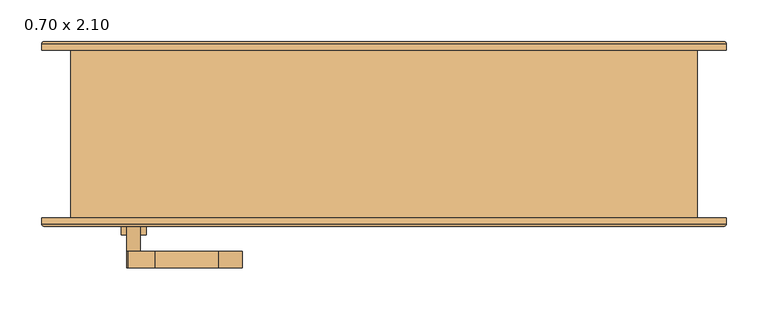
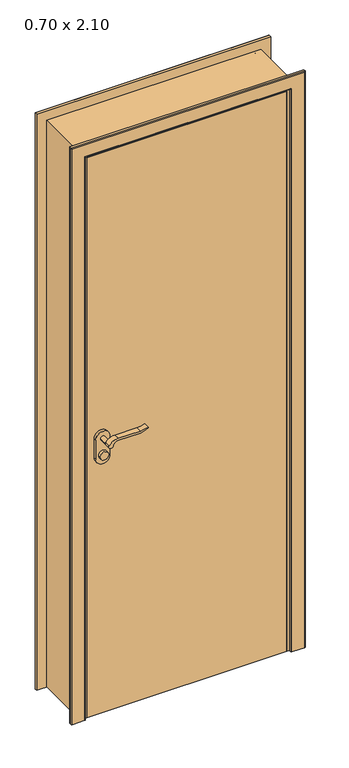
"""IFC4 building model written with IfcOpenShell, lengths in millimetres: door geometry, .CC_ND 300_PORTA SIMPLES DE ABRIR_COM EXTENSÃO : 0.70 x 2.10."""

from ifc_helpers import new_model, si_unit, point, frame, frame_2d, origin, origin_with_axes, place, context, project, spatial, polyline, circle_curve, ellipse_curve, trimmed, segment, composite_curve, outline, extrude, faceted_brep, source, transform, mapped, element, save
from ifc_brep_helpers import plane_surface, cylinder_surface, advanced_brep


def door_0_70_x_2_10_a26e7348(model_context):
    return source(origin(), model_context, "Body", "SolidModel", [
        extrude(outline(composite_curve([segment(trimmed(circle_curve(frame_2d((964.5, -300.0)), 15.0), [point((964.5, -285.0))], [point((964.5, -315.0))], False, "CARTESIAN"), True, "CONTINUOUS"), segment(trimmed(circle_curve(frame_2d((964.5, -300.0)), 15.0), [point((964.5, -315.0))], [point((964.5, -285.0))], False, "CARTESIAN"), True, "CONTINUOUS")], self_intersect=False)), frame((0.0, -120.7, 0.0), z_axis=(0.0, 1.0, 0.0), x_axis=(0.0, 0.0, 1.0)), (0.0, 0.0, 1.0), 10.0),
        extrude(outline(composite_curve([segment(trimmed(circle_curve(frame_2d((964.5, -300.0)), 15.0), [point((964.5, -285.0))], [point((964.5, -315.0))], False, "CARTESIAN"), True, "CONTINUOUS"), segment(trimmed(circle_curve(frame_2d((964.5, -300.0)), 15.0), [point((964.5, -315.0))], [point((964.5, -285.0))], False, "CARTESIAN"), True, "CONTINUOUS")], self_intersect=False)), frame((0.0, -60.7, 0.0), z_axis=(0.0, 1.0, 0.0), x_axis=(0.0, 0.0, 1.0)), (0.0, 0.0, 1.0), 10.0),
        extrude(outline(composite_curve([segment(trimmed(circle_curve(frame_2d((1024.5, -300.0)), 8.0), [point((1029.1523287, -306.5081363))], [point((1024.5, -292.0))], False, "CARTESIAN"), True, "CONTINUOUS"), segment(trimmed(circle_curve(frame_2d((1019.3738613, -274.6138099)), 18.1261387), [point((1024.5, -292.0))], [point((1037.5, -274.6138099))], True, "CARTESIAN"), True, "CONTINUOUS"), segment(polyline([(1037.5, -274.6138099), (1037.5, -198.3564091)]), True, "CONTINUOUS"), segment(trimmed(circle_curve(frame_2d((1096.7709207, -201.9396612)), 59.3791355), [point((1037.5, -198.3564091))], [point((1046.7135558, -170.0))], False, "CARTESIAN"), True, "CONTINUOUS"), segment(polyline([(1046.7135558, -170.0), (1049.5, -170.0)]), True, "CONTINUOUS"), segment(trimmed(circle_curve(frame_2d((1127.7850638, -198.4227909)), 83.2850902), [point((1049.5, -170.0))], [point((1044.5, -198.3564091))], True, "CARTESIAN"), True, "CONTINUOUS"), segment(polyline([(1044.5, -198.3564091), (1044.5, -274.6325667)]), True, "CONTINUOUS"), segment(trimmed(circle_curve(frame_2d((1007.2555521, -276.3324871)), 37.2832219), [point((1044.5, -274.6325667))], [point((1029.1523287, -306.5081363))], False, "CARTESIAN"), True, "CONTINUOUS")], self_intersect=False)), frame((0.0, -160.7, 0.0), z_axis=(0.0, 1.0, 0.0), x_axis=(0.0, 0.0, 1.0)), (0.0, 0.0, 1.0), 20.0),
        extrude(outline(composite_curve([segment(trimmed(circle_curve(frame_2d((1019.3738682, -274.6138122)), 18.1261318), [point((1024.4999903, -292.0))], [point((1037.5, -274.6138122))], True, "CARTESIAN"), True, "CONTINUOUS"), segment(polyline([(1037.5, -274.6138122), (1037.5, -198.3564091)]), True, "CONTINUOUS"), segment(trimmed(circle_curve(frame_2d((1096.7709207, -201.9396612)), 59.3791355), [point((1037.5, -198.3564091))], [point((1046.7135558, -170.0))], False, "CARTESIAN"), True, "CONTINUOUS"), segment(polyline([(1046.7135558, -170.0), (1049.5, -170.0)]), True, "CONTINUOUS"), segment(trimmed(circle_curve(frame_2d((1127.7850638, -198.4227909)), 83.2850902), [point((1049.5, -170.0))], [point((1044.5, -198.3564091))], True, "CARTESIAN"), True, "CONTINUOUS"), segment(polyline([(1044.5, -198.3564091), (1044.5, -274.6325667)]), True, "CONTINUOUS"), segment(trimmed(circle_curve(frame_2d((1007.2555521, -276.3324871)), 37.2832219), [point((1044.5, -274.6325667))], [point((1029.1523287, -306.5081363))], False, "CARTESIAN"), True, "CONTINUOUS"), segment(trimmed(circle_curve(frame_2d((1024.5, -300.0)), 8.0), [point((1029.1523287, -306.5081363))], [point((1024.4999903, -292.0))], False, "CARTESIAN"), True, "CONTINUOUS")], self_intersect=False)), frame((0.0, -30.7, 0.0), z_axis=(0.0, 1.0, 0.0), x_axis=(0.0, 0.0, 1.0)), (0.0, 0.0, 1.0), 20.0),
        extrude(outline(composite_curve([segment(trimmed(circle_curve(frame_2d((1024.5, -300.0)), 8.0), [point((1024.5, -292.0))], [point((1024.5, -308.0))], False, "CARTESIAN"), True, "CONTINUOUS"), segment(trimmed(circle_curve(frame_2d((1024.5, -300.0)), 8.0), [point((1024.5, -308.0))], [point((1024.5, -292.0))], False, "CARTESIAN"), True, "CONTINUOUS")], self_intersect=False)), frame((0.0, -140.7, 0.0), z_axis=(0.0, 1.0, 0.0), x_axis=(0.0, 0.0, 1.0)), (0.0, 0.0, 1.0), 30.0),
        extrude(outline(composite_curve([segment(trimmed(circle_curve(frame_2d((1024.5, -300.0)), 8.0), [point((1024.5, -292.0))], [point((1024.5, -308.0))], False, "CARTESIAN"), True, "CONTINUOUS"), segment(trimmed(circle_curve(frame_2d((1024.5, -300.0)), 8.0), [point((1024.5, -308.0))], [point((1024.5, -292.0))], False, "CARTESIAN"), True, "CONTINUOUS")], self_intersect=False)), frame((0.0, -60.7, 0.0), z_axis=(0.0, 1.0, 0.0), x_axis=(0.0, 0.0, 1.0)), (0.0, 0.0, 1.0), 30.0),
        extrude(outline(composite_curve([segment(trimmed(circle_curve(frame_2d((954.5, -300.0)), 25.0), [point((954.5, -325.0))], [point((954.5, -275.0))], False, "CARTESIAN"), True, "CONTINUOUS"), segment(polyline([(954.5, -275.0), (1024.5, -275.0)]), True, "CONTINUOUS"), segment(trimmed(circle_curve(frame_2d((1024.5, -300.0)), 25.0), [point((1024.5, -275.0))], [point((1024.5, -325.0))], False, "CARTESIAN"), True, "CONTINUOUS"), segment(polyline([(1024.5, -325.0), (954.5, -325.0)]), True, "CONTINUOUS")], self_intersect=False)), frame((0.0, -110.7, 0.0), z_axis=(0.0, 1.0, 0.0), x_axis=(0.0, 0.0, 1.0)), (0.0, 0.0, 1.0), 10.0),
        extrude(outline(composite_curve([segment(trimmed(circle_curve(frame_2d((954.5, -300.0)), 25.0), [point((954.5, -325.0))], [point((954.5, -275.0))], False, "CARTESIAN"), True, "CONTINUOUS"), segment(polyline([(954.5, -275.0), (1024.5, -275.0)]), True, "CONTINUOUS"), segment(trimmed(circle_curve(frame_2d((1024.5, -300.0)), 25.0), [point((1024.5, -275.0))], [point((1024.5, -325.0))], False, "CARTESIAN"), True, "CONTINUOUS"), segment(polyline([(1024.5, -325.0), (954.5, -325.0)]), True, "CONTINUOUS")], self_intersect=False)), frame((0.0, -70.7, 0.0), z_axis=(0.0, 1.0, 0.0), x_axis=(0.0, 0.0, 1.0)), (0.0, 0.0, 1.0), 10.0),
        advanced_brep(
        [(-410.0, -100.7, 0.0), (-360.0, -100.7, 0.0), (-360.0, -107.7, 0.0), (-363.0, -110.7, 0.0), (-407.0, -110.7, 0.0), (-410.0, -107.7, 0.0), (-410.0, -100.7, 2135.0), (410.0, -100.7, 2135.0), (410.0, -100.7, 0.0), (360.0, -100.7, 0.0), (360.0, -100.7, 2085.0), (-360.0, -100.7, 2085.0), (-360.0, -107.7, 2085.0), (-363.0, -110.7, 2088.0), (363.0, -110.7, 2088.0), (363.0, -110.7, 0.0), (407.0, -110.7, 0.0), (407.0, -110.7, 2132.0), (-407.0, -110.7, 2132.0), (-410.0, -107.7, 2135.0), (410.0, -107.7, 2135.0), (410.0, -107.7, 0.0), (360.0, -107.7, 0.0), (360.0, -107.7, 2085.0)],
        [
            (0, 1),
            (1, 2),
            (2, 3, circle_curve(frame((-363.0, -107.7, 0.0), z_axis=(0.0, 0.0, -1.0), x_axis=(1.0, 0.0, 0.0)), 3.0)),
            (3, 4),
            (4, 5, circle_curve(frame((-407.0, -107.7, 0.0), z_axis=(0.0, 0.0, -1.0), x_axis=(1.0, 0.0, 0.0)), 3.0)),
            (5, 0),
            (0, 6),
            (6, 7),
            (7, 8),
            (8, 9),
            (9, 10),
            (10, 11),
            (11, 1),
            (11, 12),
            (12, 2),
            (12, 13, ellipse_curve(frame((-363.0, -107.7, 2088.0), z_axis=(-0.7071067811865475, 0.0, -0.7071067811865475), x_axis=(0.7071067811865474, 0.0, -0.7071067811865476)), 4.2426407, 3.0)),
            (13, 3),
            (13, 14),
            (14, 15),
            (15, 16),
            (16, 17),
            (17, 18),
            (18, 4),
            (18, 19, ellipse_curve(frame((-407.0, -107.7, 2132.0), z_axis=(-0.7071067811865475, 0.0, -0.7071067811865475), x_axis=(0.7071067811865474, 0.0, -0.7071067811865476)), 4.2426407, 3.0)),
            (19, 5),
            (19, 6),
            (7, 20),
            (20, 21),
            (21, 8),
            (21, 16, circle_curve(frame((407.0, -107.7, 0.0), z_axis=(0.0, 0.0, -1.0), x_axis=(-1.0, 0.0, 0.0)), 3.0)),
            (15, 22, circle_curve(frame((363.0, -107.7, 0.0), z_axis=(0.0, 0.0, -1.0), x_axis=(-1.0, 0.0, 0.0)), 3.0)),
            (22, 9),
            (23, 10),
            (22, 23),
            (14, 23, ellipse_curve(frame((363.0, -107.7, 2088.0), z_axis=(0.7071067811865475, 0.0, -0.7071067811865475), x_axis=(0.7071067811865474, 0.0, 0.7071067811865476)), 4.2426407, 3.0)),
            (20, 17, ellipse_curve(frame((407.0, -107.7, 2132.0), z_axis=(0.7071067811865475, 0.0, -0.7071067811865475), x_axis=(0.7071067811865474, 0.0, 0.7071067811865476)), 4.2426407, 3.0)),
            (23, 12),
            (19, 20),
        ],
        [
            plane_surface(frame((-360.0, -100.7, 0.0), z_axis=(0.0, 0.0, -1.0), x_axis=(0.0, 1.0, 0.0))),
            plane_surface(frame((-410.0, -100.7, 0.0), z_axis=(0.0, 1.0, 0.0), x_axis=(0.0, 0.0, 1.0))),
            plane_surface(frame((-360.0, -100.7, 0.0), z_axis=(1.0, 0.0, 0.0), x_axis=(0.0, 0.0, 1.0))),
            cylinder_surface(frame((-363.0, -107.7, 0.0), z_axis=(0.0, 0.0, -1.0), x_axis=(1.0, 0.0, 0.0)), 3.0),
            plane_surface(frame((-363.0, -110.7, 0.0), z_axis=(0.0, -1.0, 0.0), x_axis=(0.0, 0.0, 1.0))),
            cylinder_surface(frame((-407.0, -107.7, 0.0), z_axis=(0.0, 0.0, -1.0), x_axis=(1.0, 0.0, 0.0)), 3.0),
            plane_surface(frame((-410.0, -107.7, 0.0), z_axis=(-1.0, 0.0, 0.0), x_axis=(0.0, 0.0, 1.0))),
            plane_surface(frame((410.0, -107.7, 2135.0), z_axis=(1.0, 0.0, 0.0), x_axis=(0.0, 0.0, -1.0))),
            plane_surface(frame((360.0, -100.7, 0.0), z_axis=(0.0, 0.0, -1.0), x_axis=(0.0, 1.0, 0.0))),
            plane_surface(frame((360.0, -100.7, 2085.0), z_axis=(-1.0, 0.0, 0.0), x_axis=(0.0, 0.0, -1.0))),
            cylinder_surface(frame((363.0, -107.7, 2085.0), z_axis=(0.0, 0.0, 1.0), x_axis=(-1.0, 0.0, 0.0)), 3.0),
            cylinder_surface(frame((407.0, -107.7, 2085.0), z_axis=(0.0, 0.0, 1.0), x_axis=(-1.0, 0.0, 0.0)), 3.0),
            plane_surface(frame((-360.0, -100.7, 2085.0), z_axis=(0.0, 0.0, -1.0), x_axis=(1.0, 0.0, 0.0))),
            plane_surface(frame((-410.0, -107.7, 2135.0), z_axis=(0.0, 0.0, 1.0), x_axis=(1.0, 0.0, 0.0))),
            cylinder_surface(frame((-360.0, -107.7, 2088.0), z_axis=(-1.0, 0.0, 0.0), x_axis=(0.0, 0.0, -1.0)), 3.0),
            cylinder_surface(frame((-360.0, -107.7, 2132.0), z_axis=(-1.0, 0.0, 0.0), x_axis=(0.0, 0.0, -1.0)), 3.0),
        ],
        [
            (0, [[1, 2, 3, 4, 5, 6]]),
            (1, [[-1, 7, 8, 9, 10, 11, 12, 13]]),
            (2, [[-2, -13, 14, 15]]),
            (3, [[-3, -15, 16, 17]]),
            (4, [[-4, -17, 18, 19, 20, 21, 22, 23]]),
            (5, [[-5, -23, 24, 25]]),
            (6, [[-6, -25, 26, -7]]),
            (7, [[27, 28, 29, -9]]),
            (8, [[-29, 30, -20, 31, 32, -10]]),
            (9, [[33, -11, -32, 34]]),
            (10, [[35, -34, -31, -19]]),
            (11, [[36, -21, -30, -28]]),
            (12, [[-14, -12, -33, 37]]),
            (13, [[-26, 38, -27, -8]]),
            (14, [[-16, -37, -35, -18]]),
            (15, [[-24, -22, -36, -38]]),
        ],
    ),
        advanced_brep(
        [(410.0, 100.7, 0.0), (360.0, 100.7, 0.0), (360.0, 107.7157283, 0.0), (362.9842717, 110.7, 0.0), (407.0342217, 110.7, 0.0), (410.0, 107.7342217, 0.0), (410.0, 100.7, 2135.0), (-410.0, 100.7, 2135.0), (-410.0, 100.7, 0.0), (-360.0, 100.7, 0.0), (-360.0, 100.7, 2085.0), (360.0, 100.7, 2085.0), (360.0, 107.7157283, 2085.0), (362.9842717, 110.7, 2087.9842717), (-362.9842717, 110.7, 2087.9842717), (-362.9842717, 110.7, 0.0), (-407.0342217, 110.7, 0.0), (-407.0342217, 110.7, 2132.0342217), (407.0342217, 110.7, 2132.0342217), (410.0, 107.7342217, 2135.0), (-410.0, 107.7342217, 2135.0), (-410.0, 107.7342217, 0.0), (-360.0, 107.7157283, 0.0), (-360.0, 107.7157283, 2085.0)],
        [
            (0, 1),
            (1, 2),
            (2, 3, circle_curve(frame((362.9842717, 107.7157283, 0.0), z_axis=(0.0, 0.0, -1.0), x_axis=(1.0, 0.0, 0.0)), 2.9842717)),
            (3, 4),
            (4, 5, circle_curve(frame((407.0342217, 107.7342217, 0.0), z_axis=(0.0, 0.0, -1.0), x_axis=(1.0, 0.0, 0.0)), 2.9657783)),
            (5, 0),
            (0, 6),
            (6, 7),
            (7, 8),
            (8, 9),
            (9, 10),
            (10, 11),
            (11, 1),
            (11, 12),
            (12, 2),
            (12, 13, ellipse_curve(frame((362.9842717, 107.7157283, 2087.9842717), z_axis=(0.7071067811865475, 0.0, -0.7071067811865475), x_axis=(-0.7071067811865474, 0.0, -0.7071067811865476)), 4.2203975, 2.9842717)),
            (13, 3),
            (13, 14),
            (14, 15),
            (15, 16),
            (16, 17),
            (17, 18),
            (18, 4),
            (18, 19, ellipse_curve(frame((407.0342217, 107.7342217, 2132.0342217), z_axis=(0.7071067811865475, 0.0, -0.7071067811865475), x_axis=(-0.7071067811865474, 0.0, -0.7071067811865476)), 4.1942438, 2.9657783)),
            (19, 5),
            (19, 6),
            (7, 20),
            (20, 21),
            (21, 8),
            (21, 16, circle_curve(frame((-407.0342217, 107.7342217, 0.0), z_axis=(0.0, 0.0, -1.0), x_axis=(-1.0, 0.0, 0.0)), 2.9657783)),
            (15, 22, circle_curve(frame((-362.9842717, 107.7157283, 0.0), z_axis=(0.0, 0.0, -1.0), x_axis=(-1.0, 0.0, 0.0)), 2.9842717)),
            (22, 9),
            (23, 10),
            (22, 23),
            (14, 23, ellipse_curve(frame((-362.9842717, 107.7157283, 2087.9842717), z_axis=(-0.7071067811865475, 0.0, -0.7071067811865475), x_axis=(-0.7071067811865474, 0.0, 0.7071067811865476)), 4.2203975, 2.9842717)),
            (20, 17, ellipse_curve(frame((-407.0342217, 107.7342217, 2132.0342217), z_axis=(-0.7071067811865475, 0.0, -0.7071067811865475), x_axis=(-0.7071067811865474, 0.0, 0.7071067811865476)), 4.1942438, 2.9657783)),
            (23, 12),
            (19, 20),
        ],
        [
            plane_surface(frame((360.0, 100.7, 0.0), z_axis=(0.0, 0.0, -1.0), x_axis=(0.0, 1.0, 0.0))),
            plane_surface(frame((410.0, 100.7, 0.0), z_axis=(0.0, -1.0, 0.0), x_axis=(0.0, 0.0, 1.0))),
            plane_surface(frame((360.0, 100.7, 0.0), z_axis=(-1.0, 0.0, 0.0), x_axis=(0.0, 0.0, 1.0))),
            cylinder_surface(frame((362.9842717, 107.7157283, 0.0), z_axis=(0.0, 0.0, -1.0), x_axis=(1.0, 0.0, 0.0)), 2.9842717),
            plane_surface(frame((362.9842717, 110.7, 0.0), z_axis=(0.0, 1.0, 0.0), x_axis=(0.0, 0.0, 1.0))),
            cylinder_surface(frame((407.0342217, 107.7342217, 0.0), z_axis=(0.0, 0.0, -1.0), x_axis=(1.0, 0.0, 0.0)), 2.9657783),
            plane_surface(frame((410.0, 107.7342217, 0.0), z_axis=(1.0, 0.0, 0.0), x_axis=(0.0, 0.0, 1.0))),
            plane_surface(frame((-410.0, 107.7342217, 2135.0), z_axis=(-1.0, 0.0, 0.0), x_axis=(0.0, 0.0, -1.0))),
            plane_surface(frame((-360.0, 100.7, 0.0), z_axis=(0.0, 0.0, -1.0), x_axis=(0.0, 1.0, 0.0))),
            plane_surface(frame((-360.0, 100.7, 2085.0), z_axis=(1.0, 0.0, 0.0), x_axis=(0.0, 0.0, -1.0))),
            cylinder_surface(frame((-362.9842717, 107.7157283, 2085.0), z_axis=(0.0, 0.0, 1.0), x_axis=(-1.0, 0.0, 0.0)), 2.9842717),
            cylinder_surface(frame((-407.0342217, 107.7342217, 2085.0), z_axis=(0.0, 0.0, 1.0), x_axis=(-1.0, 0.0, 0.0)), 2.9657783),
            plane_surface(frame((360.0, 100.7, 2085.0), z_axis=(0.0, 0.0, -1.0), x_axis=(-1.0, 0.0, 0.0))),
            plane_surface(frame((410.0, 107.7342217, 2135.0), z_axis=(0.0, 0.0, 1.0), x_axis=(-1.0, 0.0, 0.0))),
            cylinder_surface(frame((360.0, 107.7157283, 2087.9842717), z_axis=(1.0, 0.0, 0.0), x_axis=(0.0, 0.0, 1.0)), 2.9842717),
            cylinder_surface(frame((360.0, 107.7342217, 2132.0342217), z_axis=(1.0, 0.0, 0.0), x_axis=(0.0, 0.0, 1.0)), 2.9657783),
        ],
        [
            (0, [[1, 2, 3, 4, 5, 6]]),
            (1, [[-1, 7, 8, 9, 10, 11, 12, 13]]),
            (2, [[-2, -13, 14, 15]]),
            (3, [[-3, -15, 16, 17]]),
            (4, [[-4, -17, 18, 19, 20, 21, 22, 23]]),
            (5, [[-5, -23, 24, 25]]),
            (6, [[-6, -25, 26, -7]]),
            (7, [[27, 28, 29, -9]]),
            (8, [[-29, 30, -20, 31, 32, -10]]),
            (9, [[33, -11, -32, 34]]),
            (10, [[35, -34, -31, -19]]),
            (11, [[36, -21, -30, -28]]),
            (12, [[-14, -12, -33, 37]]),
            (13, [[-26, 38, -27, -8]]),
            (14, [[-16, -37, -35, -18]]),
            (15, [[-24, -22, -36, -38]]),
        ],
    ),
        faceted_brep([(342.0, 100.7, 0.0), (375.0, 100.7, 0.0), (375.0, -100.7, 0.0), (350.0, -100.7, 0.0), (350.0, -70.7, 0.0), (342.0, -70.7, 0.0), (342.0, 100.7, 2067.0), (-342.0, 100.7, 2067.0), (-342.0, 100.7, 0.0), (-375.0, 100.7, 0.0), (-375.0, 100.7, 2100.0), (375.0, 100.7, 2100.0), (375.0, -100.7, 2100.0), (-375.0, -100.7, 2100.0), (-375.0, -100.7, 0.0), (-350.0, -100.7, 0.0), (-350.0, -100.7, 2075.0), (350.0, -100.7, 2075.0), (350.0, -70.7, 2075.0), (-350.0, -70.7, 2075.0), (-350.0, -70.7, 0.0), (-342.0, -70.7, 0.0), (-342.0, -70.7, 2067.0), (342.0, -70.7, 2067.0)], [[[0, 1, 2, 3, 4, 5]], [[1, 0, 6, 7, 8, 9, 10, 11]], [[2, 1, 11, 12]], [[3, 2, 12, 13, 14, 15, 16, 17]], [[4, 3, 17, 18]], [[5, 4, 18, 19, 20, 21, 22, 23]], [[0, 5, 23, 6]], [[7, 22, 21, 8]], [[8, 21, 20, 15, 14, 9]], [[13, 10, 9, 14]], [[19, 16, 15, 20]], [[12, 11, 10, 13]], [[18, 17, 16, 19]], [[6, 23, 22, 7]]]),
        extrude(outline(polyline([(-350.0, -70.7), (350.0, -70.7), (350.0, -100.7), (-350.0, -100.7), (-350.0, -70.7)])), origin_with_axes(), (0.0, 0.0, 1.0), 2075.0),
    ])


if __name__ == "__main__":
    model = new_model("IFC4")
    model_context = context("Model", 3, world=origin())
    ifc_project = project(units=[si_unit("LENGTHUNIT", "METRE", prefix="MILLI")], contexts=[model_context])
    site = spatial("IfcSite", under=ifc_project)
    building = spatial("IfcBuilding", under=site)
    placement = place(None, origin())
    door_0_70_x_2_10_shape = door_0_70_x_2_10_a26e7348(model_context)
    element("IfcDoor", 1, ObjectType=".CC_ND 300_PORTA SIMPLES DE ABRIR_COM EXTENSÃO : 0.70 x 2.10", at=placement, inside=building, context=model_context, shape_type="MappedRepresentation", body=[
        mapped(door_0_70_x_2_10_shape, transform((0.0, 0.0, 0.0), x_axis=(1.0, 0.0, 0.0), y_axis=(0.0, 1.0, 0.0), z_axis=(0.0, 0.0, 1.0))),
    ])
    save(model, "model.ifc")

# Revit data of these elements
# Type ".CC_ND 300_PORTA SIMPLES DE ABRIR_COM EXTENSÃO : 0.70 x 2.10"
#   Type Mark = "155"
#   Rough Width = 0.75 m
#   Espessura moldura externa = 0.01 m
#   Espessura moldura interna = 0.01 m
#   Largura moldura = 0.05 m
#   Extensão acabamento exterior [instance default] = 0.00 m
#   Extensão acabamento interior [instance default] = 0.00 m
#   Espessura batente = 0.025 m
#   Thickness = 0.03 m
#   Altura batente = 2.085 m
#   Aux Arco [instance default] = 0.70 m
#   Rough Height = 2.125 m
#   Height = 2.10 m
#   Width = 0.70 m
#   Moldura interna [instance default] = yes
#   Moldura externa [instance default] = yes
#   Porta = .MADEIRA COM PINTURA ESMALTE BRANCO ACETINADO
#   Moldura = .MADEIRA COM PINTURA ESMALTE BRANCO ACETINADO
#   Maçaneta = .ALUMÍNIO
#   Batente = .MADEIRA COM PINTURA ESMALTE BRANCO ACETINADO
#   Function = (empty or 0)
#   Wall Closure = (empty or 0)
# Element 1 (IfcDoor, ".CC_ND 300_PORTA SIMPLES DE ABRIR_COM EXTENSÃO : 0.70 x 2.10")
#   Extensão acabamento exterior = 0.0257 m
#   Extensão acabamento interior = 0.0257 m
#   Aux Arco = 0.7257 m
#   Materials on its faces: ".MADEIRA COM PINTURA ESMALTE BRANCO ACETINADO", ".ALUMÍNIO"
# Materials
#   ".MADEIRA COM PINTURA ESMALTE BRANCO ACETINADO": class ".CC_MADEIRAS", colour RGB 240 240 240, transparency 0, Description = "Madeira com pintura esmalte branco acetinado.", Cost = 0
#   ".ALUMÍNIO": class "CC_METAIS", colour RGB 244 244 244, transparency 0, Description = "Material alumínio", Cost = 0
